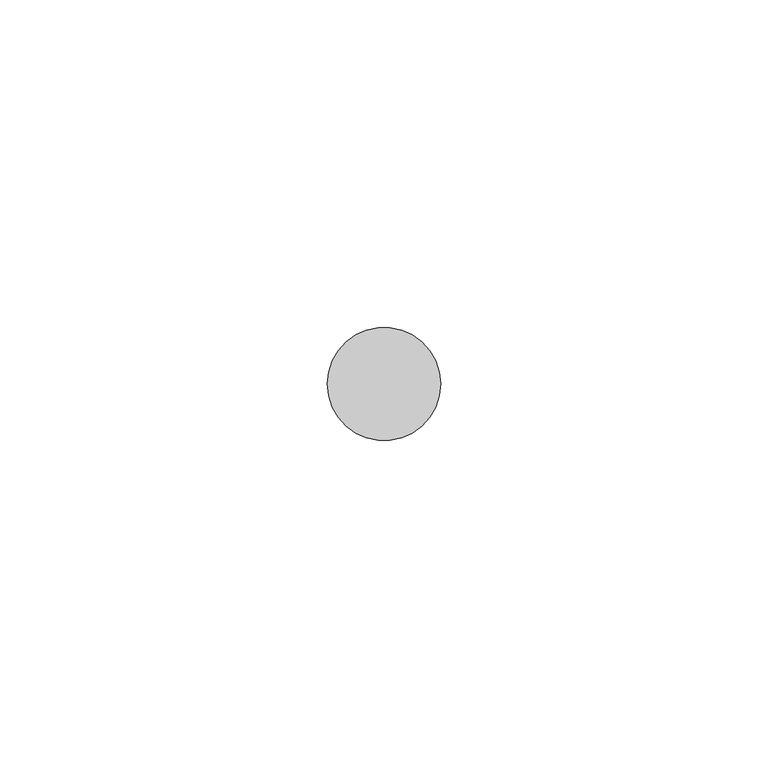
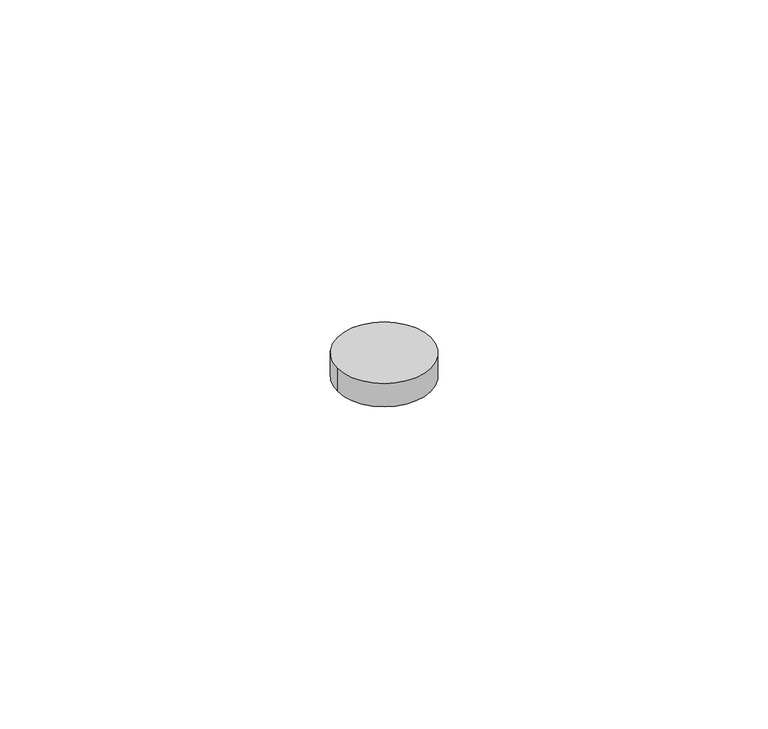
"""IFC4 building model written with IfcOpenShell, lengths in millimetres: proxy geometry, Hinge Pin Keeper4 : Hinge Pin Keeper."""

import ifcopenshell
import ifcopenshell.guid

model = None  # the IFC model being written
_history = None  # IfcOwnerHistory: only IFC2X3 demands one
_inside = {}  # id of a spatial element -> (the spatial element, [elements in it])
_under = {}  # id of a project, library or spatial element -> (it, [spatial elements below it])
_declared = {}  # id of a project -> (the project, [libraries it declares])
_typed = {}  # id of a type object -> (the type object, [elements of that type])
_made_of = {}  # id of a material, layer set ... -> (it, [elements and type objects made of it])


def new_model(schema):
    """Start an empty IFC model of exactly this schema.

    Asked for "IFC4X3", IfcOpenShell would pick the latest addendum, in which some entities
    have other attributes; the version numbers below select the first issue.
    IFC2X3 requires an IfcOwnerHistory on every rooted entity: one is made here for all.
    """
    global model, _history
    if schema == "IFC4X3":
        model = ifcopenshell.file(schema_version=(4, 3, 0, 0))
    else:
        model = ifcopenshell.file(schema=schema)
    _inside.clear()
    _under.clear()
    _declared.clear()
    _typed.clear()
    _made_of.clear()
    _history = None
    if model.schema == "IFC2X3":
        org = make("IfcOrganization", Name="unknown")
        user = make(
            "IfcPersonAndOrganization",
            ThePerson=make("IfcPerson", FamilyName="unknown"),
            TheOrganization=org,
        )
        app = make(
            "IfcApplication",
            ApplicationDeveloper=org,
            Version="unknown",
            ApplicationFullName="unknown",
            ApplicationIdentifier="unknown",
        )
        _history = make(
            "IfcOwnerHistory",
            OwningUser=user,
            OwningApplication=app,
            ChangeAction="ADDED",
            CreationDate=0,
        )
    return model


def make(cls, **values):
    """One entity of the class cls with the attributes given. An attribute that is None is left unset."""
    return model.create_entity(
        cls, **{name: value for name, value in values.items() if value is not None}
    )


def rooted(cls, **values):
    """An entity with a GlobalId (a new one), such as an element, a storey or a relation."""
    return make(cls, GlobalId=ifcopenshell.guid.new(), OwnerHistory=_history, **values)


def si_unit(unit_type, name, prefix=None):
    """IfcSIUnit, for example si_unit("LENGTHUNIT", "METRE", prefix="MILLI")."""
    return make("IfcSIUnit", UnitType=unit_type, Prefix=prefix, Name=name)


def assignment(units):
    """IfcUnitAssignment: the units of a project."""
    return None if units is None else make("IfcUnitAssignment", Units=units)


def point(xyz):
    """IfcCartesianPoint."""
    return None if xyz is None else make("IfcCartesianPoint", Coordinates=xyz)


def direction(xyz):
    """IfcDirection."""
    return None if xyz is None else make("IfcDirection", DirectionRatios=xyz)


def frame(location, z_axis=None, x_axis=None):
    """IfcAxis2Placement3D, a coordinate frame: its origin and axes. An axis left out is left unset."""
    return make(
        "IfcAxis2Placement3D",
        Location=point(location),
        Axis=direction(z_axis),
        RefDirection=direction(x_axis),
    )


def frame_2d(location, x_axis=None):
    """IfcAxis2Placement2D, a coordinate frame in the plane: its origin and x axis."""
    return make(
        "IfcAxis2Placement2D", Location=point(location), RefDirection=direction(x_axis)
    )


def origin():
    """The frame at (0, 0, 0) with its axes left unset."""
    return frame((0.0, 0.0, 0.0))


def place(relative_to, where):
    """IfcLocalPlacement: puts the frame where relative to a parent placement (None: the world)."""
    return make(
        "IfcLocalPlacement", PlacementRelTo=relative_to, RelativePlacement=where
    )


def context(
    kind, dimensions, precision=None, world=None, true_north=None, identifier=None
):
    """IfcGeometricRepresentationContext, for example the 3D "Model" context."""
    return make(
        "IfcGeometricRepresentationContext",
        ContextIdentifier=identifier,
        ContextType=kind,
        CoordinateSpaceDimension=dimensions,
        Precision=precision,
        WorldCoordinateSystem=world,
        TrueNorth=true_north,
    )


def project(units=None, contexts=None):
    """IfcProject with its units and contexts."""
    return rooted(
        "IfcProject",
        Name="project",
        RepresentationContexts=contexts,
        UnitsInContext=assignment(units),
    )


def spatial(cls, under=None, at=None, **own):
    """A site, building, storey or space (cls), placed at a placement, below another one or the project."""
    s = rooted(cls, ObjectPlacement=at, **own)
    if under is not None:
        _under.setdefault(under.id(), (under, []))[1].append(s)
    return s


def circle_curve(where, radius):
    """IfcCircle in the frame where."""
    return make("IfcCircle", Position=where, Radius=radius)


def trimmed(basis, trim1, trim2, sense, master):
    """IfcTrimmedCurve: the piece of a basis curve between two trims."""
    return make(
        "IfcTrimmedCurve",
        BasisCurve=basis,
        Trim1=trim1,
        Trim2=trim2,
        SenseAgreement=sense,
        MasterRepresentation=master,
    )


def segment(curve, same_sense, transition):
    """IfcCompositeCurveSegment."""
    return make(
        "IfcCompositeCurveSegment",
        Transition=transition,
        SameSense=same_sense,
        ParentCurve=curve,
    )


def composite_curve(segments, self_intersect=None):
    """IfcCompositeCurve: segments joined end to end."""
    return make("IfcCompositeCurve", Segments=segments, SelfIntersect=self_intersect)


def outline(outer, holes=None, kind="AREA"):
    """IfcArbitraryClosedProfileDef: a profile drawn as a closed curve; with holes, ...WithVoids."""
    if holes is None:
        return make("IfcArbitraryClosedProfileDef", ProfileType=kind, OuterCurve=outer)
    return make(
        "IfcArbitraryProfileDefWithVoids",
        ProfileType=kind,
        OuterCurve=outer,
        InnerCurves=holes,
    )


def extrude(swept, where, along, depth):
    """IfcExtrudedAreaSolid: the profile swept, set in the frame where, extruded along a direction by depth."""
    return make(
        "IfcExtrudedAreaSolid",
        SweptArea=swept,
        Position=where,
        ExtrudedDirection=direction(along),
        Depth=depth,
    )


def shape(context_of_items, identifier, shape_type, items):
    """IfcShapeRepresentation: the items that make up one representation, for example the "Body"."""
    return make(
        "IfcShapeRepresentation",
        ContextOfItems=context_of_items,
        RepresentationIdentifier=identifier,
        RepresentationType=shape_type,
        Items=items,
    )


def source(mapping_origin, context_of_items, identifier, shape_type, items):
    """IfcRepresentationMap: a shape defined once, which mapped items show again and again."""
    return make(
        "IfcRepresentationMap",
        MappingOrigin=mapping_origin,
        MappedRepresentation=shape(context_of_items, identifier, shape_type, items),
    )


def transform(
    local_origin,
    x_axis=None,
    y_axis=None,
    z_axis=None,
    scale=None,
    scale2=None,
    scale3=None,
    uniform=True,
):
    """IfcCartesianTransformationOperator3D, or its non-uniform kind. x_axis, y_axis, z_axis: its Axis1, 2, 3."""
    if uniform:
        return make(
            "IfcCartesianTransformationOperator3D",
            Axis1=direction(x_axis),
            Axis2=direction(y_axis),
            LocalOrigin=point(local_origin),
            Scale=scale,
            Axis3=direction(z_axis),
        )
    return make(
        "IfcCartesianTransformationOperator3DnonUniform",
        Axis1=direction(x_axis),
        Axis2=direction(y_axis),
        LocalOrigin=point(local_origin),
        Scale=scale,
        Axis3=direction(z_axis),
        Scale2=scale2,
        Scale3=scale3,
    )


def mapped(mapping_source, mapping_target):
    """IfcMappedItem: shows the shape of a source again, moved by a transform."""
    return make(
        "IfcMappedItem", MappingSource=mapping_source, MappingTarget=mapping_target
    )


def made_of(thing, what):
    """Note that an element or type object is made of a material, layer set ...; save() writes the relation."""
    if what is not None:
        _made_of.setdefault(what.id(), (what, []))[1].append(thing)
    return thing


def element(
    cls,
    number,
    at=None,
    inside=None,
    cuts=None,
    type_object=None,
    material=None,
    context=None,
    identifier="Body",
    shape_type=None,
    held_by="IfcProductDefinitionShape",
    body=None,
    shapes=None,
    **own,
):
    """One element of the class cls, such as IfcWall. Its Tag is "e" and its number.

    at: its placement. inside: the storey or other place that contains it. cuts: it is an
    opening in that element (IfcRelVoidsElement). A single representation is given by context,
    identifier, shape_type and body (its items); several are given by shapes. held_by: the class
    of the entity that holds the representations. save() writes the other relations.
    """
    e = rooted(cls, Tag="e%d" % number, ObjectPlacement=at, **own)
    if body is not None:
        shapes = [shape(context, identifier, shape_type, body)]
    if shapes is not None:
        e.Representation = make(held_by, Representations=shapes)
    if inside is not None:
        _inside.setdefault(inside.id(), (inside, []))[1].append(e)
    if cuts is not None:
        rooted(
            "IfcRelVoidsElement", RelatingBuildingElement=cuts, RelatedOpeningElement=e
        )
    if type_object is not None:
        _typed.setdefault(type_object.id(), (type_object, []))[1].append(e)
    return made_of(e, material)


def aggregate(whole, parts):
    """IfcRelAggregates: a whole, such as a stair, and the parts it consists of."""
    return rooted("IfcRelAggregates", RelatingObject=whole, RelatedObjects=parts)


def save(model, path):
    """Write the relations noted so far, then the file.

    IfcRelAggregates (storeys below a building ...), IfcRelContainedInSpatialStructure (elements
    in a storey), IfcRelDefinesByType, IfcRelAssociatesMaterial and IfcRelDeclares: one each for
    every whole, place, type object, material and project.
    """
    for whole, parts in _under.values():
        aggregate(whole, parts)
    for where, things in _inside.values():
        rooted(
            "IfcRelContainedInSpatialStructure",
            RelatedElements=things,
            RelatingStructure=where,
        )
    for kind, things in _typed.values():
        rooted("IfcRelDefinesByType", RelatedObjects=things, RelatingType=kind)
    for what, things in _made_of.values():
        rooted("IfcRelAssociatesMaterial", RelatedObjects=things, RelatingMaterial=what)
    for by, libraries in _declared.values():
        rooted("IfcRelDeclares", RelatingContext=by, RelatedDefinitions=libraries)
    model.write(path)


def generic_models_80a38197(model_context):
    return source(origin(), model_context, "Body", "SweptSolid", [
        extrude(outline(composite_curve([segment(trimmed(circle_curve(frame_2d((587319.1320739, -531776.6049841)), 8.6534625), [point((587310.4786114, -531776.6049841))], [point((587327.7855364, -531776.6049841))], False, "CARTESIAN"), True, "CONTINUOUS"), segment(trimmed(circle_curve(frame_2d((587319.1320739, -531776.6049841)), 8.6534625), [point((587327.7855364, -531776.6049841))], [point((587310.4786114, -531776.6049841))], False, "CARTESIAN"), True, "CONTINUOUS")], self_intersect=False)), frame((0.0, 0.0, 1271.7859375), z_axis=(0.0, 0.0, 1.0), x_axis=(1.0, 0.0, 0.0)), (0.0, 0.0, 1.0), 4.5640625),
    ])


if __name__ == "__main__":
    model = new_model("IFC4")
    model_context = context("Model", 3, world=origin())
    ifc_project = project(units=[si_unit("LENGTHUNIT", "METRE", prefix="MILLI")], contexts=[model_context])
    site = spatial("IfcSite", under=ifc_project)
    building = spatial("IfcBuilding", under=site)
    placement = place(None, origin())
    generic_models_shape = generic_models_80a38197(model_context)
    element("IfcBuildingElementProxy", 1, Name="Hinge Pin Keeper4 : Hinge Pin Keeper", ObjectType="Hinge Pin Keeper4 : Hinge Pin Keeper", at=placement, inside=building, context=model_context, shape_type="MappedRepresentation", body=[
        mapped(generic_models_shape, transform((0.0, 0.0, 0.0), x_axis=(1.0, 0.0, 0.0), y_axis=(0.0, 1.0, 0.0), z_axis=(0.0, 0.0, 1.0))),
    ])
    save(model, "model.ifc")

# Revit data of these elements
# Element 1 (IfcBuildingElementProxy, "Hinge Pin Keeper4 : Hinge Pin Keeper")
#   Materials on its faces: "6\"X6\" WELD-ON STL BUTT HINGE"
# Materials
#   "6\"X6\" WELD-ON STL BUTT HINGE": class "Metal", colour RGB 189 187 185, transparency 0, Description = "Carbon steel", Cost = 0
